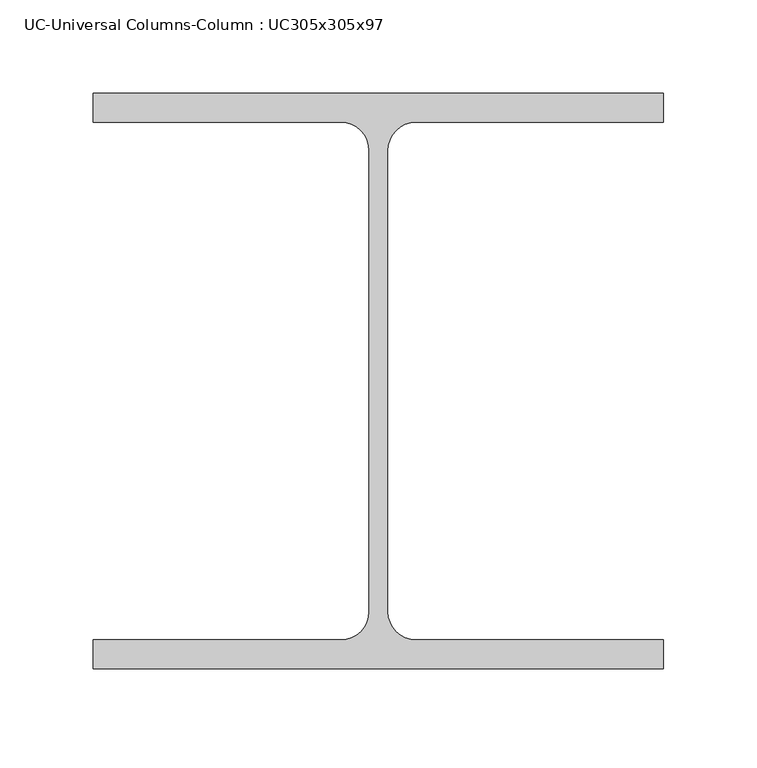
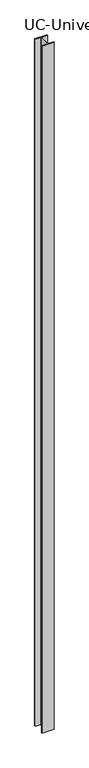
"""IFC4 building model written with IfcOpenShell, lengths in millimetres: column geometry, UC-Universal Columns-Column : UC305x305x97."""

from ifc_helpers import new_model, si_unit, point, frame, frame_2d, origin, place, context, project, spatial, polyline, circle_curve, trimmed, segment, composite_curve, outline, extrude, source, transform, mapped, element, save


def uc_universal_columns_column_uc305x305x97_e2fb10fc(model_context):
    return source(origin(), model_context, "Body", "SweptSolid", [
        extrude(outline(composite_curve([segment(polyline([(152.65, 153.95), (152.65, 138.55), (20.15, 138.55)]), True, "CONTINUOUS"), segment(trimmed(circle_curve(frame_2d((20.15, 123.35)), 15.2), [point((20.15, 138.55))], [point((4.95, 123.35))], True, "CARTESIAN"), True, "CONTINUOUS"), segment(polyline([(4.95, 123.35), (4.95, -123.35)]), True, "CONTINUOUS"), segment(trimmed(circle_curve(frame_2d((20.15, -123.35)), 15.2), [point((4.95, -123.35))], [point((20.15, -138.55))], True, "CARTESIAN"), True, "CONTINUOUS"), segment(polyline([(20.15, -138.55), (152.65, -138.55), (152.65, -153.95), (-152.65, -153.95), (-152.65, -138.55), (-20.15, -138.55)]), True, "CONTINUOUS"), segment(trimmed(circle_curve(frame_2d((-20.15, -123.35)), 15.2), [point((-20.15, -138.55))], [point((-4.95, -123.35))], True, "CARTESIAN"), True, "CONTINUOUS"), segment(polyline([(-4.95, -123.35), (-4.95, 123.35)]), True, "CONTINUOUS"), segment(trimmed(circle_curve(frame_2d((-20.15, 123.35)), 15.2), [point((-4.95, 123.35))], [point((-20.15, 138.55))], True, "CARTESIAN"), True, "CONTINUOUS"), segment(polyline([(-20.15, 138.55), (-152.65, 138.55), (-152.65, 153.95), (152.65, 153.95)]), True, "CONTINUOUS")], self_intersect=False)), frame((0.0, 0.0, -5550.0), z_axis=(0.0, 0.0, 1.0), x_axis=(1.0, 0.0, 0.0)), (0.0, 0.0, 1.0), 17989.0),
    ])


if __name__ == "__main__":
    model = new_model("IFC4")
    model_context = context("Model", 3, world=origin())
    ifc_project = project(units=[si_unit("LENGTHUNIT", "METRE", prefix="MILLI")], contexts=[model_context])
    site = spatial("IfcSite", under=ifc_project)
    building = spatial("IfcBuilding", under=site)
    placement = place(None, origin())
    uc_universal_columns_column_uc305x305x97_shape = uc_universal_columns_column_uc305x305x97_e2fb10fc(model_context)
    element("IfcColumn", 1, ObjectType="UC-Universal Columns-Column : UC305x305x97", at=placement, inside=building, context=model_context, shape_type="MappedRepresentation", body=[
        mapped(uc_universal_columns_column_uc305x305x97_shape, transform((0.0, 0.0, 0.0), x_axis=(1.0, 0.0, 0.0), y_axis=(0.0, 1.0, 0.0), z_axis=(0.0, 0.0, 1.0))),
    ])
    save(model, "model.ifc")

# Revit data of these elements
# Type "UC-Universal Columns-Column : UC305x305x97"
#   Section Name Key = "UC305x305x97"
#   Cost = 2
#   Width = 30.53 cm
#   Web Thickness = 0.99 cm
#   Web Fillet = 1.52 cm
#   Warping Constant = 1560000.0 cm⁶
#   Torsional Moment of Inertia = 91.20 cm⁴
#   Section Area = 123.0 cm²
#   Plastic Modulus weak axis = 726.0 cm³
#   Plastic Modulus strong axis = 1592.0 cm³
#   Nominal Weight = 96.8996 kgf/m
#   Moment of Inertia weak axis = 7308.00 cm⁴
#   Moment of Inertia strong axis = 22249.00 cm⁴
#   Height = 30.79 cm
#   Flange Thickness = 1.54 cm
#   Elastic Modulus weak axis = 479.0 cm³
#   Elastic Modulus strong axis = 1445.0 cm³
#   Centroid Vertical = 15.395 cm
#   Centroid Horizontal = 15.265 cm
#   Bolt Spacing = 14.0 cm
#   Structural Material [instance default] = Metal - Steel 43-275
#   Type Comments = ""
#   Assembly Code = ""
# Element 1 (IfcColumn, "UC-Universal Columns-Column : UC305x305x97")
#   Materials on its faces: "Metal - Steel 43-275"
# Materials
#   "Metal - Steel 43-275": class "Metal", colour RGB 247 247 247, transparency 0, Cost = 0
